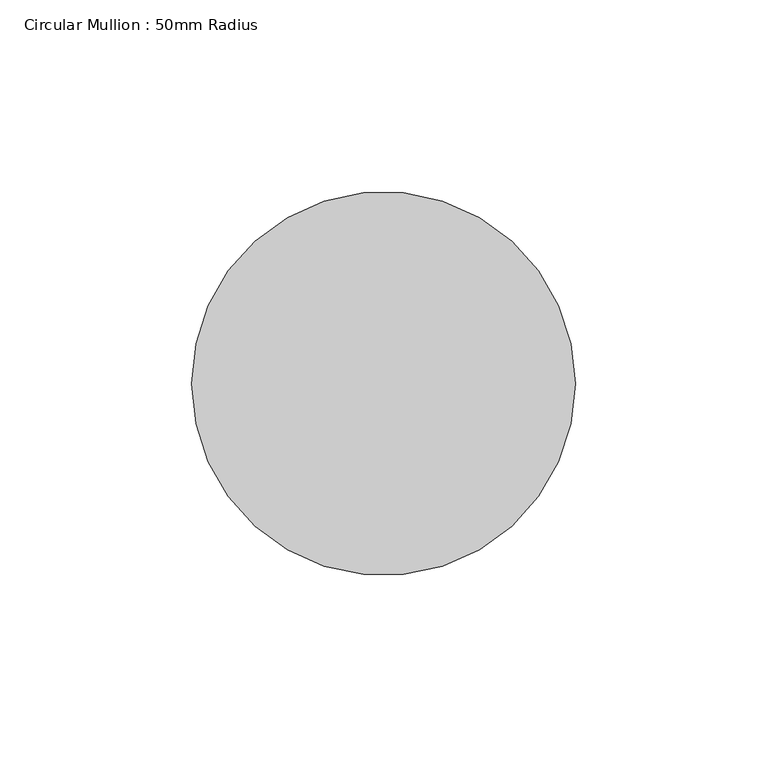
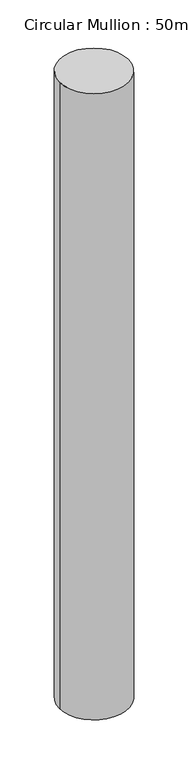
"""IFC4 building model written with IfcOpenShell, lengths in millimetres: member geometry, Circular Mullion : 50mm Radius."""

from ifc_helpers import new_model, si_unit, point, frame, origin, origin_2d, place, context, project, spatial, circle_curve, trimmed, segment, composite_curve, outline, extrude, source, transform, mapped, element, save


def circular_mullion_50mm_radius_c340cd98(model_context):
    return source(origin(), model_context, "Body", "SweptSolid", [
        extrude(outline(composite_curve([segment(trimmed(circle_curve(origin_2d(), 50.0), [point((50.0, 0.0))], [point((-50.0, 0.0))], False, "CARTESIAN"), True, "CONTINUOUS"), segment(trimmed(circle_curve(origin_2d(), 50.0), [point((-50.0, 0.0))], [point((50.0, 0.0))], False, "CARTESIAN"), True, "CONTINUOUS")], self_intersect=False)), frame((0.0, 0.0, -963.2908775), z_axis=(0.0, 0.0, 1.0), x_axis=(1.0, 0.0, 0.0)), (0.0, 0.0, 1.0), 963.2908775),
    ])


if __name__ == "__main__":
    model = new_model("IFC4")
    model_context = context("Model", 3, world=origin())
    ifc_project = project(units=[si_unit("LENGTHUNIT", "METRE", prefix="MILLI")], contexts=[model_context])
    site = spatial("IfcSite", under=ifc_project)
    building = spatial("IfcBuilding", under=site)
    placement = place(None, origin())
    circular_mullion_50mm_radius_shape = circular_mullion_50mm_radius_c340cd98(model_context)
    element("IfcMember", 1, ObjectType="Circular Mullion : 50mm Radius", at=placement, inside=building, context=model_context, shape_type="MappedRepresentation", body=[
        mapped(circular_mullion_50mm_radius_shape, transform((0.0, 0.0, 0.0), x_axis=(1.0, 0.0, 0.0), y_axis=(0.0, 1.0, 0.0), z_axis=(0.0, 0.0, 1.0))),
    ])
    save(model, "model.ifc")

# Revit data of these elements
# Type "Circular Mullion : 50mm Radius"
#   built-in parameter 1007350 = 0.164042 (stored number, unit not read)
# Element 1 (IfcMember, "Circular Mullion : 50mm Radius")
#   Materials on its faces: "Aluminium"
# Materials
#   "Aluminium": class "Metal", colour RGB 247 247 247, transparency 0, Description = "Aluminium 6061", Cost = 0
